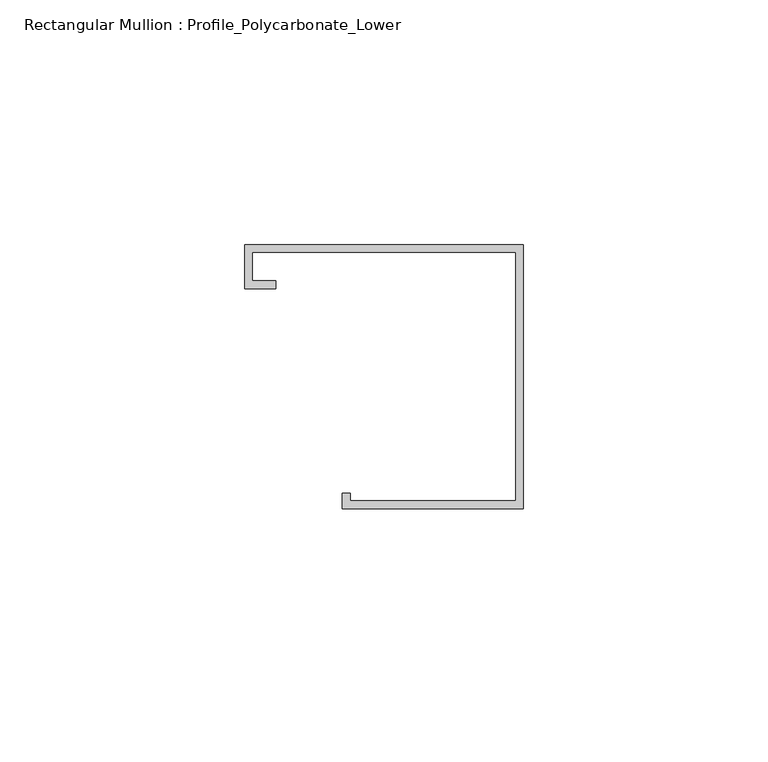
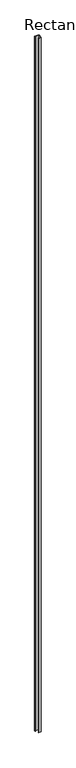
"""IFC4 building model written with IfcOpenShell, lengths in millimetres: member geometry, Rectangular Mullion : Profile_Polycarbonate_Lower."""

from ifc_helpers import new_model, si_unit, frame, origin, place, context, project, spatial, polyline, outline, extrude, source, transform, mapped, element, save


def rectangular_mullion_profile_polycarbonate_lower_192744ab(model_context):
    return source(origin(), model_context, "Body", "SweptSolid", [
        extrude(outline(polyline([(0.0, 28.984575), (0.0, -25.015825), (-36.9824, -25.015825), (-36.9824, -21.840825), (-35.3949, -21.840825), (-35.3949, -23.428325), (-1.5875, -23.428325), (-1.5875, 27.397075), (-55.4101, 27.397075), (-55.4101, 21.580475), (-50.6476, 21.580475), (-50.6476, 19.992975), (-56.9976, 19.992975), (-56.9976, 28.984575), (0.0, 28.984575)])), frame((0.0, 0.0, -9863.2899), z_axis=(0.0, 0.0, 1.0), x_axis=(1.0, 0.0, 0.0)), (0.0, 0.0, 1.0), 9863.2899),
    ])


if __name__ == "__main__":
    model = new_model("IFC4")
    model_context = context("Model", 3, world=origin())
    ifc_project = project(units=[si_unit("LENGTHUNIT", "METRE", prefix="MILLI")], contexts=[model_context])
    site = spatial("IfcSite", under=ifc_project)
    building = spatial("IfcBuilding", under=site)
    placement = place(None, origin())
    rectangular_mullion_profile_polycarbonate_lower_shape = rectangular_mullion_profile_polycarbonate_lower_192744ab(model_context)
    element("IfcMember", 1, ObjectType="Rectangular Mullion : Profile_Polycarbonate_Lower", at=placement, inside=building, context=model_context, shape_type="MappedRepresentation", body=[
        mapped(rectangular_mullion_profile_polycarbonate_lower_shape, transform((0.0, 0.0, 0.0), x_axis=(1.0, 0.0, 0.0), y_axis=(0.0, 1.0, 0.0), z_axis=(0.0, 0.0, 1.0))),
    ])
    save(model, "model.ifc")

# Revit data of these elements
# Type "Rectangular Mullion : Profile_Polycarbonate_Lower"
#   built-in parameter 1007322 = 0.177167 (stored number, unit not read)
#   built-in parameter 1007321 = 0 (stored number, unit not read)
#   built-in parameter 1007320 = 0.00520833 (stored number, unit not read)
